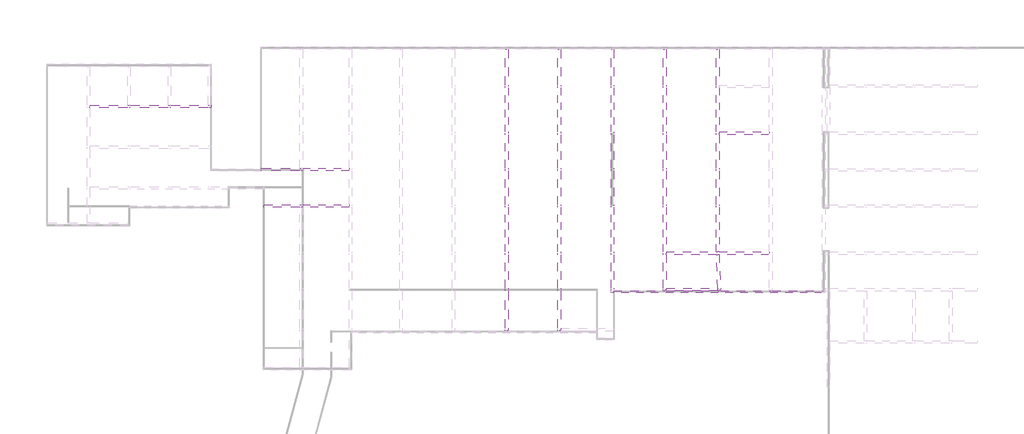
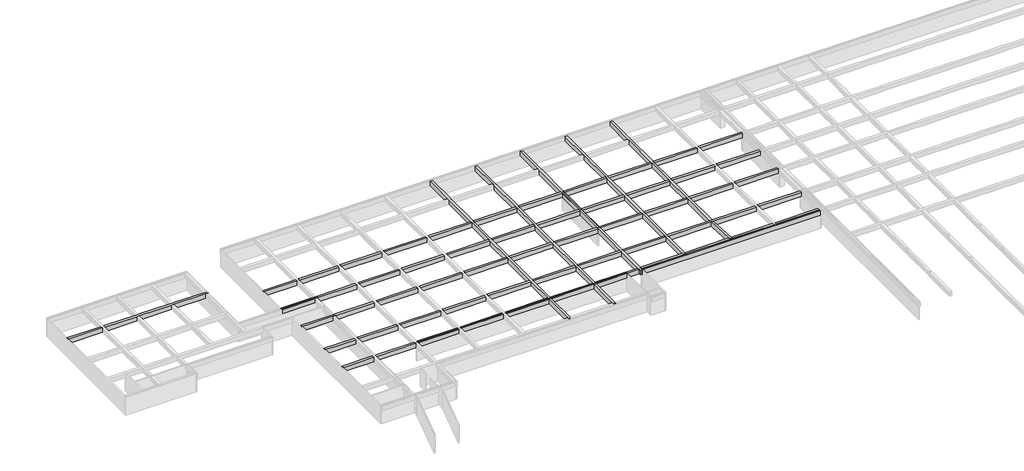
# One storey, part 5 of 14: 13 beams.
"""IFC4 building model written with IfcOpenShell, lengths in millimetres."""

from ifc_helpers import new_model, si_unit, frame, origin, place, context, project, spatial, polyline, outline, extrude, faceted_brep, element, save

model = new_model("IFC4")

# Units and contexts
model_context = context("Model", 3, world=origin())
ifc_project = project(units=[si_unit("LENGTHUNIT", "METRE", prefix="MILLI")], contexts=[model_context])

# Site, building, storey
site = spatial("IfcSite", under=ifc_project)
building = spatial("IfcBuilding", under=site)
storey = spatial("IfcBuildingStorey", under=building, Name="户型图", Elevation=0.0)

# Beams
placement = place(None, origin())
element("IfcBeam", 1, ObjectType="混凝土 - 矩形梁 : KL_beam", at=placement, inside=storey, context=model_context, shape_type="Brep", body=[
    faceted_brep([(-77750.8485237, -125836.5894684, 3300.0), (-77750.8485237, -126236.5894684, 3300.0), (-77750.8485237, -126236.5894684, 2500.0), (-77750.8485237, -125836.5894684, 2500.0), (-77800.8485237, -125836.5894684, 3300.0), (-78200.8485237, -125836.5894684, 3300.0), (-83675.8485237, -125836.5894684, 3300.0), (-84075.8485237, -125836.5894684, 3300.0), (-89675.8485237, -125836.5894684, 3300.0), (-90075.8485237, -125836.5894684, 3300.0), (-95664.0025134, -125836.5894684, 3300.0), (-95664.0025134, -126236.5894684, 3300.0), (-90075.8485237, -126236.5894684, 3300.0), (-89675.8485237, -126236.5894684, 3300.0), (-84075.8485237, -126236.5894684, 3300.0), (-83675.8485237, -126236.5894684, 3300.0), (-78200.8485237, -126236.5894684, 3300.0), (-77800.8485237, -126236.5894684, 3300.0), (-95664.0025134, -126236.5894684, 2500.0), (-90075.8485237, -126236.5894684, 2500.0), (-89675.8485237, -126236.5894684, 2500.0), (-84075.8485237, -126236.5894684, 2500.0), (-83675.8485237, -126236.5894684, 2500.0), (-78200.8485237, -126236.5894684, 2500.0), (-77800.8485237, -126236.5894684, 2500.0), (-95664.0025134, -125836.5894684, 2500.0), (-90075.8485237, -125836.5894684, 2500.0), (-89675.8485237, -125836.5894684, 2500.0), (-84075.8485237, -125836.5894684, 2500.0), (-83675.8485237, -125836.5894684, 2500.0), (-78200.8485237, -125836.5894684, 2500.0), (-77800.8485237, -125836.5894684, 2500.0)], [[[0, 1, 2, 3]], [[1, 0, 4, 5, 6, 7, 8, 9, 10, 11, 12, 13, 14, 15, 16, 17]], [[2, 1, 17, 16, 15, 14, 13, 12, 11, 18, 19, 20, 21, 22, 23, 24]], [[3, 2, 24, 23, 22, 21, 20, 19, 18, 25, 26, 27, 28, 29, 30, 31]], [[0, 3, 31, 30, 29, 28, 27, 26, 25, 10, 9, 8, 7, 6, 5, 4]], [[11, 10, 25, 18]]]),
    faceted_brep([(-102000.8485237, -125836.5894684, 3300.0), (-102000.8485237, -125836.5894684, 2500.0), (-102000.8485237, -126236.5894684, 2500.0), (-102000.8485237, -126236.5894684, 3300.0), (-96064.0025134, -125836.5894684, 3300.0), (-96064.0025134, -126236.5894684, 3300.0), (-96064.0025134, -126236.5894684, 2500.0), (-96064.0025134, -125836.5894684, 2500.0)], [[[0, 1, 2, 3]], [[4, 5, 6, 7]], [[0, 3, 5, 4]], [[3, 2, 6, 5]], [[2, 1, 7, 6]], [[1, 0, 4, 7]]]),
])
element("IfcBeam", 2, ObjectType="混凝土 - 矩形梁 : KL_beam", at=placement, inside=storey, context=model_context, shape_type="Brep", body=[
    faceted_brep([(-34272.7050956, -159158.4277999, 3300.0), (-33872.7050956, -159158.4277999, 3300.0), (-33872.7050956, -158807.3751505, 3300.0), (-33872.7050956, -153248.950757, 3300.0), (-33872.7050956, -152848.950757, 3300.0), (-33872.7050956, -147899.284307, 3300.0), (-33872.7050956, -147499.284307, 3300.0), (-33872.7050956, -140920.0179086, 3300.0), (-33872.7050956, -140520.0179086, 3300.0), (-33872.7050956, -135526.4975491, 3300.0), (-33872.7050956, -135126.4975491, 3300.0), (-33872.7050956, -130180.0179086, 3300.0), (-33872.7050956, -129780.0179086, 3300.0), (-33872.7050956, -123258.950757, 3300.0), (-33872.7050956, -122858.950757, 3300.0), (-33872.7050956, -117558.950757, 3300.0), (-34272.7050956, -117558.950757, 3300.0), (-34272.7050956, -122858.950757, 3300.0), (-34272.7050956, -123258.950757, 3300.0), (-34272.7050956, -129780.0179086, 3300.0), (-34272.7050956, -130180.0179086, 3300.0), (-34272.7050956, -135126.4975491, 3300.0), (-34272.7050956, -135526.4975491, 3300.0), (-34272.7050956, -140520.0179086, 3300.0), (-34272.7050956, -140920.0179086, 3300.0), (-34272.7050956, -147499.284307, 3300.0), (-34272.7050956, -147899.284307, 3300.0), (-34272.7050956, -152848.950757, 3300.0), (-34272.7050956, -153248.950757, 3300.0), (-34272.7050956, -158807.3751505, 3300.0), (-34272.7050956, -159158.4277999, 2500.0), (-34272.7050956, -117558.950757, 2500.0), (-34272.7050956, -122858.950757, 2500.0), (-34272.7050956, -123258.950757, 2500.0), (-34272.7050956, -129780.0179086, 2500.0), (-34272.7050956, -130180.0179086, 2500.0), (-34272.7050956, -135126.4975491, 2500.0), (-34272.7050956, -135526.4975491, 2500.0), (-34272.7050956, -140520.0179086, 2500.0), (-34272.7050956, -140920.0179086, 2500.0), (-34272.7050956, -147499.284307, 2500.0), (-34272.7050956, -147899.284307, 2500.0), (-34272.7050956, -152848.950757, 2500.0), (-34272.7050956, -153248.950757, 2500.0), (-34272.7050956, -158807.3751505, 2500.0), (-33872.7050956, -159158.4277999, 2500.0), (-33872.7050956, -117558.950757, 2500.0), (-33872.7050956, -122858.950757, 2500.0), (-33872.7050956, -123258.950757, 2500.0), (-33872.7050956, -129780.0179086, 2500.0), (-33872.7050956, -130180.0179086, 2500.0), (-33872.7050956, -135126.4975491, 2500.0), (-33872.7050956, -135526.4975491, 2500.0), (-33872.7050956, -140520.0179086, 2500.0), (-33872.7050956, -140920.0179086, 2500.0), (-33872.7050956, -147499.284307, 2500.0), (-33872.7050956, -147899.284307, 2500.0), (-33872.7050956, -152848.950757, 2500.0), (-33872.7050956, -153248.950757, 2500.0), (-33872.7050956, -158807.3751505, 2500.0)], [[[0, 1, 2, 3, 4, 5, 6, 7, 8, 9, 10, 11, 12, 13, 14, 15, 16, 17, 18, 19, 20, 21, 22, 23, 24, 25, 26, 27, 28, 29]], [[30, 0, 29, 28, 27, 26, 25, 24, 23, 22, 21, 20, 19, 18, 17, 16, 31, 32, 33, 34, 35, 36, 37, 38, 39, 40, 41, 42, 43, 44]], [[45, 30, 44, 43, 42, 41, 40, 39, 38, 37, 36, 35, 34, 33, 32, 31, 46, 47, 48, 49, 50, 51, 52, 53, 54, 55, 56, 57, 58, 59]], [[1, 45, 59, 58, 57, 56, 55, 54, 53, 52, 51, 50, 49, 48, 47, 46, 15, 14, 13, 12, 11, 10, 9, 8, 7, 6, 5, 4, 3, 2]], [[1, 0, 30, 45]], [[16, 15, 46, 31]]]),
])
element("IfcBeam", 3, ObjectType="混凝土 - 矩形梁 : KL_beam", at=placement, inside=storey, context=model_context, shape_type="Brep", body=[
    faceted_brep([(-26492.7050956, -159158.4277999, 3300.0), (-26092.7050956, -159158.4277999, 3300.0), (-26092.7050956, -158807.3751505, 3300.0), (-26092.7050956, -153248.950757, 3300.0), (-26092.7050956, -152848.950757, 3300.0), (-26092.7050956, -147899.284307, 3300.0), (-26092.7050956, -147499.284307, 3300.0), (-26092.7050956, -140920.0179086, 3300.0), (-26092.7050956, -140520.0179086, 3300.0), (-26092.7050956, -135526.4975491, 3300.0), (-26092.7050956, -135126.4975491, 3300.0), (-26092.7050956, -130180.0179086, 3300.0), (-26092.7050956, -129780.0179086, 3300.0), (-26092.7050956, -123258.950757, 3300.0), (-26092.7050956, -122858.950757, 3300.0), (-26092.7050956, -117558.950757, 3300.0), (-26492.7050956, -117558.950757, 3300.0), (-26492.7050956, -122858.950757, 3300.0), (-26492.7050956, -123258.950757, 3300.0), (-26492.7050956, -129780.0179086, 3300.0), (-26492.7050956, -130180.0179086, 3300.0), (-26492.7050956, -135126.4975491, 3300.0), (-26492.7050956, -135526.4975491, 3300.0), (-26492.7050956, -140520.0179086, 3300.0), (-26492.7050956, -140920.0179086, 3300.0), (-26492.7050956, -147499.284307, 3300.0), (-26492.7050956, -147899.284307, 3300.0), (-26492.7050956, -152848.950757, 3300.0), (-26492.7050956, -153248.950757, 3300.0), (-26492.7050956, -158807.3751505, 3300.0), (-26092.7050956, -159158.4277999, 2500.0), (-26092.7050956, -158807.3751505, 2500.0), (-26092.7050956, -153248.950757, 2500.0), (-26092.7050956, -152848.950757, 2500.0), (-26092.7050956, -147899.284307, 2500.0), (-26092.7050956, -147499.284307, 2500.0), (-26092.7050956, -140920.0179086, 2500.0), (-26092.7050956, -140520.0179086, 2500.0), (-26092.7050956, -135526.4975491, 2500.0), (-26092.7050956, -135126.4975491, 2500.0), (-26092.7050956, -130180.0179086, 2500.0), (-26092.7050956, -129780.0179086, 2500.0), (-26092.7050956, -123258.950757, 2500.0), (-26092.7050956, -122858.950757, 2500.0), (-26092.7050956, -117558.950757, 2500.0), (-26492.7050956, -159158.4277999, 2500.0), (-26492.7050956, -158807.3751505, 2500.0), (-26492.7050956, -153248.950757, 2500.0), (-26492.7050956, -152848.950757, 2500.0), (-26492.7050956, -147899.284307, 2500.0), (-26492.7050956, -147499.284307, 2500.0), (-26492.7050956, -140920.0179086, 2500.0), (-26492.7050956, -140520.0179086, 2500.0), (-26492.7050956, -135526.4975491, 2500.0), (-26492.7050956, -135126.4975491, 2500.0), (-26492.7050956, -130180.0179086, 2500.0), (-26492.7050956, -129780.0179086, 2500.0), (-26492.7050956, -123258.950757, 2500.0), (-26492.7050956, -122858.950757, 2500.0), (-26492.7050956, -117558.950757, 2500.0)], [[[0, 1, 2, 3, 4, 5, 6, 7, 8, 9, 10, 11, 12, 13, 14, 15, 16, 17, 18, 19, 20, 21, 22, 23, 24, 25, 26, 27, 28, 29]], [[1, 30, 31, 32, 33, 34, 35, 36, 37, 38, 39, 40, 41, 42, 43, 44, 15, 14, 13, 12, 11, 10, 9, 8, 7, 6, 5, 4, 3, 2]], [[30, 45, 46, 47, 48, 49, 50, 51, 52, 53, 54, 55, 56, 57, 58, 59, 44, 43, 42, 41, 40, 39, 38, 37, 36, 35, 34, 33, 32, 31]], [[45, 0, 29, 28, 27, 26, 25, 24, 23, 22, 21, 20, 19, 18, 17, 16, 59, 58, 57, 56, 55, 54, 53, 52, 51, 50, 49, 48, 47, 46]], [[1, 0, 45, 30]], [[16, 15, 44, 59]]]),
])
element("IfcBeam", 4, ObjectType="混凝土 - 矩形梁 : KL_beam", at=placement, inside=storey, context=model_context, shape_type="Brep", body=[
    faceted_brep([(-18655.2993912, -153567.1629538, 3300.0), (-18255.2993912, -153567.1629538, 3300.0), (-18255.2993912, -153248.950757, 3300.0), (-18255.2993912, -152848.950757, 3300.0), (-18255.2993912, -147899.284307, 3300.0), (-18255.2993912, -147499.284307, 3300.0), (-18255.2993912, -140920.0179086, 3300.0), (-18255.2993912, -140520.0179086, 3300.0), (-18255.2993912, -135526.4975491, 3300.0), (-18255.2993912, -135126.4975491, 3300.0), (-18255.2993912, -130180.0179086, 3300.0), (-18255.2993912, -129780.0179086, 3300.0), (-18255.2993912, -123258.950757, 3300.0), (-18255.2993912, -122858.950757, 3300.0), (-18255.2993912, -117558.950757, 3300.0), (-18655.2993912, -117558.950757, 3300.0), (-18655.2993912, -122858.950757, 3300.0), (-18655.2993912, -123258.950757, 3300.0), (-18655.2993912, -129780.0179086, 3300.0), (-18655.2993912, -130180.0179086, 3300.0), (-18655.2993912, -135126.4975491, 3300.0), (-18655.2993912, -135526.4975491, 3300.0), (-18655.2993912, -140520.0179086, 3300.0), (-18655.2993912, -140920.0179086, 3300.0), (-18655.2993912, -147499.284307, 3300.0), (-18655.2993912, -147899.284307, 3300.0), (-18655.2993912, -152848.950757, 3300.0), (-18655.2993912, -153248.950757, 3300.0), (-18655.2993912, -153567.1629538, 2500.0), (-18655.2993912, -117558.950757, 2500.0), (-18655.2993912, -122858.950757, 2500.0), (-18655.2993912, -123258.950757, 2500.0), (-18655.2993912, -129780.0179086, 2500.0), (-18655.2993912, -130180.0179086, 2500.0), (-18655.2993912, -135126.4975491, 2500.0), (-18655.2993912, -135526.4975491, 2500.0), (-18655.2993912, -140520.0179086, 2500.0), (-18655.2993912, -140920.0179086, 2500.0), (-18655.2993912, -147499.284307, 2500.0), (-18655.2993912, -147899.284307, 2500.0), (-18655.2993912, -152848.950757, 2500.0), (-18655.2993912, -153248.950757, 2500.0), (-18255.2993912, -153567.1629538, 2500.0), (-18255.2993912, -117558.950757, 2500.0), (-18255.2993912, -122858.950757, 2500.0), (-18255.2993912, -123258.950757, 2500.0), (-18255.2993912, -129780.0179086, 2500.0), (-18255.2993912, -130180.0179086, 2500.0), (-18255.2993912, -135126.4975491, 2500.0), (-18255.2993912, -135526.4975491, 2500.0), (-18255.2993912, -140520.0179086, 2500.0), (-18255.2993912, -140920.0179086, 2500.0), (-18255.2993912, -147499.284307, 2500.0), (-18255.2993912, -147899.284307, 2500.0), (-18255.2993912, -152848.950757, 2500.0), (-18255.2993912, -153248.950757, 2500.0)], [[[0, 1, 2, 3, 4, 5, 6, 7, 8, 9, 10, 11, 12, 13, 14, 15, 16, 17, 18, 19, 20, 21, 22, 23, 24, 25, 26, 27]], [[28, 0, 27, 26, 25, 24, 23, 22, 21, 20, 19, 18, 17, 16, 15, 29, 30, 31, 32, 33, 34, 35, 36, 37, 38, 39, 40, 41]], [[42, 28, 41, 40, 39, 38, 37, 36, 35, 34, 33, 32, 31, 30, 29, 43, 44, 45, 46, 47, 48, 49, 50, 51, 52, 53, 54, 55]], [[1, 42, 55, 54, 53, 52, 51, 50, 49, 48, 47, 46, 45, 44, 43, 14, 13, 12, 11, 10, 9, 8, 7, 6, 5, 4, 3, 2]], [[1, 0, 28, 42]], [[15, 14, 43, 29]]]),
])
element("IfcBeam", 5, ObjectType="混凝土 - 矩形梁 : KL_beam", at=placement, inside=storey, context=model_context, shape_type="Brep", body=[
    faceted_brep([(-10914.1452268, -153167.1629538, 3300.0), (-10514.1452268, -153167.1629538, 3300.0), (-10514.1452268, -152848.950757, 3300.0), (-10514.1452268, -147899.284307, 3300.0), (-10514.1452268, -147499.284307, 3300.0), (-10514.1452268, -140920.0179086, 3300.0), (-10514.1452268, -140520.0179086, 3300.0), (-10514.1452268, -135526.4975491, 3300.0), (-10514.1452268, -135126.4975491, 3300.0), (-10514.1452268, -130180.0179086, 3300.0), (-10514.1452268, -129780.0179086, 3300.0), (-10514.1452268, -123258.950757, 3300.0), (-10514.1452268, -122858.950757, 3300.0), (-10514.1452268, -117558.950757, 3300.0), (-10914.1452268, -117558.950757, 3300.0), (-10914.1452268, -122858.950757, 3300.0), (-10914.1452268, -123258.950757, 3300.0), (-10914.1452268, -129780.0179086, 3300.0), (-10914.1452268, -130180.0179086, 3300.0), (-10914.1452268, -135126.4975491, 3300.0), (-10914.1452268, -135526.4975491, 3300.0), (-10914.1452268, -140520.0179086, 3300.0), (-10914.1452268, -140920.0179086, 3300.0), (-10914.1452268, -147499.284307, 3300.0), (-10914.1452268, -147899.284307, 3300.0), (-10914.1452268, -152848.950757, 3300.0), (-10914.1452268, -153167.1629538, 2500.0), (-10914.1452268, -117558.950757, 2500.0), (-10914.1452268, -122858.950757, 2500.0), (-10914.1452268, -123258.950757, 2500.0), (-10914.1452268, -129780.0179086, 2500.0), (-10914.1452268, -130180.0179086, 2500.0), (-10914.1452268, -135126.4975491, 2500.0), (-10914.1452268, -135526.4975491, 2500.0), (-10914.1452268, -140520.0179086, 2500.0), (-10914.1452268, -140920.0179086, 2500.0), (-10914.1452268, -147499.284307, 2500.0), (-10914.1452268, -147899.284307, 2500.0), (-10914.1452268, -152848.950757, 2500.0), (-10514.1452268, -153167.1629538, 2500.0), (-10514.1452268, -117558.950757, 2500.0), (-10514.1452268, -122858.950757, 2500.0), (-10514.1452268, -123258.950757, 2500.0), (-10514.1452268, -129780.0179086, 2500.0), (-10514.1452268, -130180.0179086, 2500.0), (-10514.1452268, -135126.4975491, 2500.0), (-10514.1452268, -135526.4975491, 2500.0), (-10514.1452268, -140520.0179086, 2500.0), (-10514.1452268, -140920.0179086, 2500.0), (-10514.1452268, -147499.284307, 2500.0), (-10514.1452268, -147899.284307, 2500.0), (-10514.1452268, -152848.950757, 2500.0)], [[[0, 1, 2, 3, 4, 5, 6, 7, 8, 9, 10, 11, 12, 13, 14, 15, 16, 17, 18, 19, 20, 21, 22, 23, 24, 25]], [[26, 0, 25, 24, 23, 22, 21, 20, 19, 18, 17, 16, 15, 14, 27, 28, 29, 30, 31, 32, 33, 34, 35, 36, 37, 38]], [[39, 26, 38, 37, 36, 35, 34, 33, 32, 31, 30, 29, 28, 27, 40, 41, 42, 43, 44, 45, 46, 47, 48, 49, 50, 51]], [[1, 39, 51, 50, 49, 48, 47, 46, 45, 44, 43, 42, 41, 40, 13, 12, 11, 10, 9, 8, 7, 6, 5, 4, 3, 2]], [[1, 0, 26, 39]], [[14, 13, 40, 27]]]),
])
element("IfcBeam", 6, ObjectType="混凝土 - 矩形梁 : KL_beam", at=placement, inside=storey, context=model_context, shape_type="Brep", body=[
    faceted_brep([(-2680.6534407, -147899.284307, 3300.0), (-3081.0325897, -147899.284307, 3300.0), (-2865.4722954, -152848.950757, 3300.0), (-2851.6140051, -153167.1629538, 3300.0), (-2451.2348561, -153167.1629538, 3300.0), (-2465.0931464, -152848.950757, 3300.0), (-2680.6534407, -147899.284307, 2500.0), (-2451.2348561, -153167.1629538, 2500.0), (-2465.0931464, -152848.950757, 2500.0), (-3081.0325897, -147899.284307, 2500.0), (-2851.6140051, -153167.1629538, 2500.0), (-2865.4722954, -152848.950757, 2500.0)], [[[0, 1, 2, 3, 4, 5]], [[6, 0, 5, 4, 7, 8]], [[9, 6, 8, 7, 10, 11]], [[1, 9, 11, 10, 3, 2]], [[1, 0, 6, 9]], [[4, 3, 10, 7]]]),
])
element("IfcBeam", 7, ObjectType="混凝土 - 矩形梁 : KL_beam", at=placement, inside=storey, context=model_context, shape_type="Brep", body=[
    faceted_brep([(-2691.5778774, -147499.284307, 3300.0), (-2691.5778774, -147499.284307, 2500.0), (-2691.5778774, -140920.0179086, 2500.0), (-2691.5778774, -140520.0179086, 2500.0), (-2691.5778774, -135526.4975491, 2500.0), (-2691.5778774, -135126.4975491, 2500.0), (-2691.5778774, -130180.0179086, 2500.0), (-2691.5778774, -129780.0179086, 2500.0), (-2691.5778774, -123258.950757, 2500.0), (-2691.5778774, -122858.950757, 2500.0), (-2691.5778774, -117558.950757, 2500.0), (-2691.5778774, -117558.950757, 3300.0), (-2691.5778774, -122858.950757, 3300.0), (-2691.5778774, -123258.950757, 3300.0), (-2691.5778774, -129780.0179086, 3300.0), (-2691.5778774, -130180.0179086, 3300.0), (-2691.5778774, -135126.4975491, 3300.0), (-2691.5778774, -135526.4975491, 3300.0), (-2691.5778774, -140520.0179086, 3300.0), (-2691.5778774, -140920.0179086, 3300.0), (-3091.5778774, -147499.284307, 3300.0), (-3091.5778774, -147499.284307, 2500.0), (-3091.5778774, -117558.950757, 3300.0), (-3091.5778774, -122858.950757, 3300.0), (-3091.5778774, -123258.950757, 3300.0), (-3091.5778774, -129780.0179086, 3300.0), (-3091.5778774, -130180.0179086, 3300.0), (-3091.5778774, -135126.4975491, 3300.0), (-3091.5778774, -135526.4975491, 3300.0), (-3091.5778774, -140520.0179086, 3300.0), (-3091.5778774, -140920.0179086, 3300.0), (-3091.5778774, -140920.0179086, 2500.0), (-3091.5778774, -140520.0179086, 2500.0), (-3091.5778774, -135526.4975491, 2500.0), (-3091.5778774, -135126.4975491, 2500.0), (-3091.5778774, -130180.0179086, 2500.0), (-3091.5778774, -129780.0179086, 2500.0), (-3091.5778774, -123258.950757, 2500.0), (-3091.5778774, -122858.950757, 2500.0), (-3091.5778774, -117558.950757, 2500.0)], [[[0, 1, 2, 3, 4, 5, 6, 7, 8, 9, 10, 11, 12, 13, 14, 15, 16, 17, 18, 19]], [[20, 21, 1, 0]], [[20, 0, 19, 18, 17, 16, 15, 14, 13, 12, 11, 22, 23, 24, 25, 26, 27, 28, 29, 30]], [[1, 21, 31, 32, 33, 34, 35, 36, 37, 38, 39, 10, 9, 8, 7, 6, 5, 4, 3, 2]], [[21, 20, 30, 29, 28, 27, 26, 25, 24, 23, 22, 39, 38, 37, 36, 35, 34, 33, 32, 31]], [[11, 10, 39, 22]]]),
])
element("IfcBeam", 8, ObjectType="混凝土 - 矩形梁 : KL_beam", at=placement, inside=storey, context=model_context, shape_type="SweptSolid", body=[
    extrude(outline(polyline([(-70372.7050956, -130180.0179086), (-70372.7050956, -129780.0179086), (-64612.7050956, -129780.0179086), (-64612.7050956, -130180.0179086), (-70372.7050956, -130180.0179086)])), frame((0.0, 0.0, 2500.0), z_axis=(0.0, 0.0, 1.0), x_axis=(1.0, 0.0, 0.0)), (0.0, 0.0, 1.0), 800.0),
    extrude(outline(polyline([(12577.2949044, -129780.0179086), (12577.2949044, -130180.0179086), (5154.7716095, -130180.0179086), (5154.7716095, -129780.0179086), (12577.2949044, -129780.0179086)])), frame((0.0, 0.0, 2500.0), z_axis=(0.0, 0.0, 1.0), x_axis=(1.0, 0.0, 0.0)), (0.0, 0.0, 1.0), 800.0),
    extrude(outline(polyline([(-64212.7050956, -130180.0179086), (-64212.7050956, -129780.0179086), (-57355.3281677, -129780.0179086), (-57355.3281677, -130180.0179086), (-64212.7050956, -130180.0179086)])), frame((0.0, 0.0, 2500.0), z_axis=(0.0, 0.0, 1.0), x_axis=(1.0, 0.0, 0.0)), (0.0, 0.0, 1.0), 800.0),
    extrude(outline(polyline([(-56955.3281677, -130180.0179086), (-56955.3281677, -129780.0179086), (-49869.9201432, -129780.0179086), (-49869.9201432, -130180.0179086), (-56955.3281677, -130180.0179086)])), frame((0.0, 0.0, 2500.0), z_axis=(0.0, 0.0, 1.0), x_axis=(1.0, 0.0, 0.0)), (0.0, 0.0, 1.0), 800.0),
    extrude(outline(polyline([(-49469.9201432, -130180.0179086), (-49469.9201432, -129780.0179086), (-42115.0194088, -129780.0179086), (-42115.0194088, -130180.0179086), (-49469.9201432, -130180.0179086)])), frame((0.0, 0.0, 2500.0), z_axis=(0.0, 0.0, 1.0), x_axis=(1.0, 0.0, 0.0)), (0.0, 0.0, 1.0), 800.0),
    extrude(outline(polyline([(-41715.0194088, -130180.0179086), (-41715.0194088, -129780.0179086), (-34272.7050956, -129780.0179086), (-34272.7050956, -130180.0179086), (-41715.0194088, -130180.0179086)])), frame((0.0, 0.0, 2500.0), z_axis=(0.0, 0.0, 1.0), x_axis=(1.0, 0.0, 0.0)), (0.0, 0.0, 1.0), 800.0),
    extrude(outline(polyline([(-33872.7050956, -130180.0179086), (-33872.7050956, -129780.0179086), (-26492.7050956, -129780.0179086), (-26492.7050956, -130180.0179086), (-33872.7050956, -130180.0179086)])), frame((0.0, 0.0, 2500.0), z_axis=(0.0, 0.0, 1.0), x_axis=(1.0, 0.0, 0.0)), (0.0, 0.0, 1.0), 800.0),
    extrude(outline(polyline([(-26092.7050956, -130180.0179086), (-26092.7050956, -129780.0179086), (-18655.2993912, -129780.0179086), (-18655.2993912, -130180.0179086), (-26092.7050956, -130180.0179086)])), frame((0.0, 0.0, 2500.0), z_axis=(0.0, 0.0, 1.0), x_axis=(1.0, 0.0, 0.0)), (0.0, 0.0, 1.0), 800.0),
    extrude(outline(polyline([(-18255.2993912, -130180.0179086), (-18255.2993912, -129780.0179086), (-10914.1452268, -129780.0179086), (-10914.1452268, -130180.0179086), (-18255.2993912, -130180.0179086)])), frame((0.0, 0.0, 2500.0), z_axis=(0.0, 0.0, 1.0), x_axis=(1.0, 0.0, 0.0)), (0.0, 0.0, 1.0), 800.0),
    extrude(outline(polyline([(-10514.1452268, -130180.0179086), (-10514.1452268, -129780.0179086), (-3091.5778774, -129780.0179086), (-3091.5778774, -130180.0179086), (-10514.1452268, -130180.0179086)])), frame((0.0, 0.0, 2500.0), z_axis=(0.0, 0.0, 1.0), x_axis=(1.0, 0.0, 0.0)), (0.0, 0.0, 1.0), 800.0),
    extrude(outline(polyline([(-2691.5778774, -130180.0179086), (-2691.5778774, -129780.0179086), (4754.7716095, -129780.0179086), (4754.7716095, -130180.0179086), (-2691.5778774, -130180.0179086)])), frame((0.0, 0.0, 2500.0), z_axis=(0.0, 0.0, 1.0), x_axis=(1.0, 0.0, 0.0)), (0.0, 0.0, 1.0), 800.0),
])
element("IfcBeam", 9, ObjectType="混凝土 - 矩形梁 : KL_beam", at=placement, inside=storey, context=model_context, shape_type="Brep", body=[
    faceted_brep([(-57355.3281677, -135126.4975491, 3300.0), (-64212.7050956, -135126.4975491, 3300.0), (-64612.7050956, -135126.4975491, 3300.0), (-70313.0159659, -135126.4975491, 3300.0), (-70313.0159659, -135208.950757, 3300.0), (-70313.0159659, -135526.4975491, 3300.0), (-64612.7050956, -135526.4975491, 3300.0), (-64212.7050956, -135526.4975491, 3300.0), (-57355.3281677, -135526.4975491, 3300.0), (-70313.0159659, -135526.4975491, 2500.0), (-64612.7050956, -135526.4975491, 2500.0), (-64212.7050956, -135526.4975491, 2500.0), (-57355.3281677, -135526.4975491, 2500.0), (-70313.0159659, -135208.950757, 2500.0), (-70313.0159659, -135126.4975491, 2500.0), (-64612.7050956, -135126.4975491, 2500.0), (-64212.7050956, -135126.4975491, 2500.0), (-57355.3281677, -135126.4975491, 2500.0)], [[[0, 1, 2, 3, 4, 5, 6, 7, 8]], [[8, 7, 6, 5, 9, 10, 11, 12]], [[12, 11, 10, 9, 13, 14, 15, 16, 17]], [[3, 2, 1, 0, 17, 16, 15, 14]], [[0, 8, 12, 17]], [[3, 14, 13, 9, 5, 4]]]),
    faceted_brep([(12577.2949044, -135126.4975491, 3300.0), (12577.2949044, -135526.4975491, 3300.0), (12577.2949044, -135526.4975491, 2500.0), (12577.2949044, -135126.4975491, 2500.0), (5154.7716095, -135526.4975491, 3300.0), (5154.7716095, -135126.4975491, 3300.0), (5154.7716095, -135126.4975491, 2500.0), (5154.7716095, -135526.4975491, 2500.0)], [[[0, 1, 2, 3]], [[4, 5, 6, 7]], [[1, 0, 5, 4]], [[2, 1, 4, 7]], [[3, 2, 7, 6]], [[0, 3, 6, 5]]]),
    faceted_brep([(-56955.3281677, -135526.4975491, 3300.0), (-56955.3281677, -135126.4975491, 3300.0), (-56955.3281677, -135126.4975491, 2500.0), (-56955.3281677, -135526.4975491, 2500.0), (-49869.9201432, -135126.4975491, 3300.0), (-49869.9201432, -135526.4975491, 3300.0), (-49869.9201432, -135526.4975491, 2500.0), (-49869.9201432, -135126.4975491, 2500.0)], [[[0, 1, 2, 3]], [[4, 5, 6, 7]], [[1, 0, 5, 4]], [[0, 3, 6, 5]], [[3, 2, 7, 6]], [[2, 1, 4, 7]]]),
    faceted_brep([(-42115.0194088, -135126.4975491, 3300.0), (-49469.9201432, -135126.4975491, 3300.0), (-49469.9201432, -135526.4975491, 3300.0), (-42115.0194088, -135526.4975491, 3300.0), (-49469.9201432, -135526.4975491, 2500.0), (-42115.0194088, -135526.4975491, 2500.0), (-49469.9201432, -135126.4975491, 2500.0), (-42115.0194088, -135126.4975491, 2500.0)], [[[0, 1, 2, 3]], [[3, 2, 4, 5]], [[5, 4, 6, 7]], [[1, 0, 7, 6]], [[2, 1, 6, 4]], [[0, 3, 5, 7]]]),
    faceted_brep([(-41715.0194088, -135526.4975491, 3300.0), (-41715.0194088, -135126.4975491, 3300.0), (-41715.0194088, -135126.4975491, 2500.0), (-41715.0194088, -135526.4975491, 2500.0), (-34272.7050956, -135126.4975491, 3300.0), (-34272.7050956, -135526.4975491, 3300.0), (-34272.7050956, -135526.4975491, 2500.0), (-34272.7050956, -135126.4975491, 2500.0)], [[[0, 1, 2, 3]], [[4, 5, 6, 7]], [[4, 1, 0, 5]], [[5, 0, 3, 6]], [[6, 3, 2, 7]], [[1, 4, 7, 2]]]),
    faceted_brep([(-33872.7050956, -135526.4975491, 3300.0), (-33872.7050956, -135126.4975491, 3300.0), (-33872.7050956, -135126.4975491, 2500.0), (-33872.7050956, -135526.4975491, 2500.0), (-26492.7050956, -135126.4975491, 3300.0), (-26492.7050956, -135526.4975491, 3300.0), (-26492.7050956, -135526.4975491, 2500.0), (-26492.7050956, -135126.4975491, 2500.0)], [[[0, 1, 2, 3]], [[4, 5, 6, 7]], [[4, 1, 0, 5]], [[5, 0, 3, 6]], [[6, 3, 2, 7]], [[1, 4, 7, 2]]]),
    faceted_brep([(-26092.7050956, -135526.4975491, 3300.0), (-26092.7050956, -135126.4975491, 3300.0), (-26092.7050956, -135126.4975491, 2500.0), (-26092.7050956, -135526.4975491, 2500.0), (-18655.2993912, -135126.4975491, 3300.0), (-18655.2993912, -135526.4975491, 3300.0), (-18655.2993912, -135526.4975491, 2500.0), (-18655.2993912, -135126.4975491, 2500.0)], [[[0, 1, 2, 3]], [[4, 5, 6, 7]], [[4, 1, 0, 5]], [[5, 0, 3, 6]], [[6, 3, 2, 7]], [[1, 4, 7, 2]]]),
    faceted_brep([(-18255.2993912, -135526.4975491, 3300.0), (-18255.2993912, -135126.4975491, 3300.0), (-18255.2993912, -135126.4975491, 2500.0), (-18255.2993912, -135526.4975491, 2500.0), (-10914.1452268, -135126.4975491, 3300.0), (-10914.1452268, -135526.4975491, 3300.0), (-10914.1452268, -135526.4975491, 2500.0), (-10914.1452268, -135126.4975491, 2500.0)], [[[0, 1, 2, 3]], [[4, 5, 6, 7]], [[4, 1, 0, 5]], [[5, 0, 3, 6]], [[6, 3, 2, 7]], [[1, 4, 7, 2]]]),
    faceted_brep([(-10514.1452268, -135526.4975491, 3300.0), (-10514.1452268, -135126.4975491, 3300.0), (-10514.1452268, -135126.4975491, 2500.0), (-10514.1452268, -135526.4975491, 2500.0), (-3091.5778774, -135126.4975491, 3300.0), (-3091.5778774, -135526.4975491, 3300.0), (-3091.5778774, -135526.4975491, 2500.0), (-3091.5778774, -135126.4975491, 2500.0)], [[[0, 1, 2, 3]], [[4, 5, 6, 7]], [[4, 1, 0, 5]], [[5, 0, 3, 6]], [[6, 3, 2, 7]], [[1, 4, 7, 2]]]),
    faceted_brep([(-2691.5778774, -135526.4975491, 3300.0), (-2691.5778774, -135126.4975491, 3300.0), (-2691.5778774, -135126.4975491, 2500.0), (-2691.5778774, -135526.4975491, 2500.0), (4754.7716095, -135126.4975491, 3300.0), (4754.7716095, -135526.4975491, 3300.0), (4754.7716095, -135526.4975491, 2500.0), (4754.7716095, -135126.4975491, 2500.0)], [[[0, 1, 2, 3]], [[4, 5, 6, 7]], [[1, 0, 5, 4]], [[0, 3, 6, 5]], [[3, 2, 7, 6]], [[2, 1, 4, 7]]]),
])
element("IfcBeam", 10, ObjectType="混凝土 - 矩形梁 : KL_beam", at=placement, inside=storey, context=model_context, shape_type="Brep", body=[
    faceted_brep([(-69972.7050956, -140920.0179086, 3300.0), (-69972.7050956, -140520.0179086, 3300.0), (-69972.7050956, -140520.0179086, 2500.0), (-69972.7050956, -140920.0179086, 2500.0), (-64612.7050956, -140920.0179086, 3300.0), (-64212.7050956, -140920.0179086, 3300.0), (-57355.3281677, -140920.0179086, 3300.0), (-57355.3281677, -140520.0179086, 3300.0), (-64212.7050956, -140520.0179086, 3300.0), (-64612.7050956, -140520.0179086, 3300.0), (-57355.3281677, -140520.0179086, 2500.0), (-64212.7050956, -140520.0179086, 2500.0), (-64612.7050956, -140520.0179086, 2500.0), (-57355.3281677, -140920.0179086, 2500.0), (-64212.7050956, -140920.0179086, 2500.0), (-64612.7050956, -140920.0179086, 2500.0)], [[[0, 1, 2, 3]], [[1, 0, 4, 5, 6, 7, 8, 9]], [[2, 1, 9, 8, 7, 10, 11, 12]], [[3, 2, 12, 11, 10, 13, 14, 15]], [[0, 3, 15, 14, 13, 6, 5, 4]], [[7, 6, 13, 10]]]),
    faceted_brep([(12577.2949044, -140520.0179086, 3300.0), (12577.2949044, -140920.0179086, 3300.0), (12577.2949044, -140920.0179086, 2500.0), (12577.2949044, -140520.0179086, 2500.0), (5154.7716095, -140920.0179086, 3300.0), (5154.7716095, -140520.0179086, 3300.0), (5154.7716095, -140520.0179086, 2500.0), (5154.7716095, -140920.0179086, 2500.0)], [[[0, 1, 2, 3]], [[4, 5, 6, 7]], [[1, 0, 5, 4]], [[0, 3, 6, 5]], [[3, 2, 7, 6]], [[2, 1, 4, 7]]]),
    faceted_brep([(-56955.3281677, -140920.0179086, 3300.0), (-56955.3281677, -140520.0179086, 3300.0), (-56955.3281677, -140520.0179086, 2500.0), (-56955.3281677, -140920.0179086, 2500.0), (-49869.9201432, -140920.0179086, 3300.0), (-49869.9201432, -140520.0179086, 3300.0), (-49869.9201432, -140520.0179086, 2500.0), (-49869.9201432, -140920.0179086, 2500.0)], [[[0, 1, 2, 3]], [[1, 0, 4, 5]], [[2, 1, 5, 6]], [[3, 2, 6, 7]], [[0, 3, 7, 4]], [[5, 4, 7, 6]]]),
    faceted_brep([(-49469.9201432, -140920.0179086, 3300.0), (-49469.9201432, -140520.0179086, 3300.0), (-49469.9201432, -140520.0179086, 2500.0), (-49469.9201432, -140920.0179086, 2500.0), (-42115.0194088, -140920.0179086, 3300.0), (-42115.0194088, -140520.0179086, 3300.0), (-42115.0194088, -140520.0179086, 2500.0), (-42115.0194088, -140920.0179086, 2500.0)], [[[0, 1, 2, 3]], [[1, 0, 4, 5]], [[2, 1, 5, 6]], [[3, 2, 6, 7]], [[0, 3, 7, 4]], [[5, 4, 7, 6]]]),
    faceted_brep([(-41715.0194088, -140920.0179086, 3300.0), (-41715.0194088, -140520.0179086, 3300.0), (-41715.0194088, -140520.0179086, 2500.0), (-41715.0194088, -140920.0179086, 2500.0), (-34272.7050956, -140920.0179086, 3300.0), (-34272.7050956, -140520.0179086, 3300.0), (-34272.7050956, -140520.0179086, 2500.0), (-34272.7050956, -140920.0179086, 2500.0)], [[[0, 1, 2, 3]], [[1, 0, 4, 5]], [[2, 1, 5, 6]], [[3, 2, 6, 7]], [[0, 3, 7, 4]], [[5, 4, 7, 6]]]),
    faceted_brep([(-33872.7050956, -140920.0179086, 3300.0), (-33872.7050956, -140520.0179086, 3300.0), (-33872.7050956, -140520.0179086, 2500.0), (-33872.7050956, -140920.0179086, 2500.0), (-26492.7050956, -140920.0179086, 3300.0), (-26492.7050956, -140520.0179086, 3300.0), (-26492.7050956, -140520.0179086, 2500.0), (-26492.7050956, -140920.0179086, 2500.0)], [[[0, 1, 2, 3]], [[1, 0, 4, 5]], [[2, 1, 5, 6]], [[3, 2, 6, 7]], [[0, 3, 7, 4]], [[5, 4, 7, 6]]]),
    faceted_brep([(-26092.7050956, -140920.0179086, 3300.0), (-26092.7050956, -140520.0179086, 3300.0), (-26092.7050956, -140520.0179086, 2500.0), (-26092.7050956, -140920.0179086, 2500.0), (-18655.2993912, -140920.0179086, 3300.0), (-18655.2993912, -140520.0179086, 3300.0), (-18655.2993912, -140520.0179086, 2500.0), (-18655.2993912, -140920.0179086, 2500.0)], [[[0, 1, 2, 3]], [[1, 0, 4, 5]], [[2, 1, 5, 6]], [[3, 2, 6, 7]], [[0, 3, 7, 4]], [[5, 4, 7, 6]]]),
    faceted_brep([(-18255.2993912, -140920.0179086, 3300.0), (-18255.2993912, -140520.0179086, 3300.0), (-18255.2993912, -140520.0179086, 2500.0), (-18255.2993912, -140920.0179086, 2500.0), (-10914.1452268, -140920.0179086, 3300.0), (-10914.1452268, -140520.0179086, 3300.0), (-10914.1452268, -140520.0179086, 2500.0), (-10914.1452268, -140920.0179086, 2500.0)], [[[0, 1, 2, 3]], [[1, 0, 4, 5]], [[2, 1, 5, 6]], [[3, 2, 6, 7]], [[0, 3, 7, 4]], [[5, 4, 7, 6]]]),
    faceted_brep([(-10514.1452268, -140920.0179086, 3300.0), (-10514.1452268, -140520.0179086, 3300.0), (-10514.1452268, -140520.0179086, 2500.0), (-10514.1452268, -140920.0179086, 2500.0), (-3091.5778774, -140920.0179086, 3300.0), (-3091.5778774, -140520.0179086, 3300.0), (-3091.5778774, -140520.0179086, 2500.0), (-3091.5778774, -140920.0179086, 2500.0)], [[[0, 1, 2, 3]], [[1, 0, 4, 5]], [[2, 1, 5, 6]], [[3, 2, 6, 7]], [[0, 3, 7, 4]], [[5, 4, 7, 6]]]),
    faceted_brep([(-2691.5778774, -140920.0179086, 3300.0), (-2691.5778774, -140520.0179086, 3300.0), (-2691.5778774, -140520.0179086, 2500.0), (-2691.5778774, -140920.0179086, 2500.0), (4754.7716095, -140920.0179086, 3300.0), (4754.7716095, -140520.0179086, 3300.0), (4754.7716095, -140520.0179086, 2500.0), (4754.7716095, -140920.0179086, 2500.0)], [[[0, 1, 2, 3]], [[1, 0, 4, 5]], [[2, 1, 5, 6]], [[3, 2, 6, 7]], [[0, 3, 7, 4]], [[5, 4, 7, 6]]]),
])
element("IfcBeam", 11, ObjectType="混凝土 - 矩形梁 : KL_beam", at=placement, inside=storey, context=model_context, shape_type="Brep", body=[
    faceted_brep([(-69972.7050956, -147499.284307, 3300.0), (-69972.7050956, -147499.284307, 2500.0), (-69972.7050956, -147899.284307, 2500.0), (-69972.7050956, -147899.284307, 3300.0), (-64612.7050956, -147499.284307, 3300.0), (-64612.7050956, -147899.284307, 3300.0), (-64612.7050956, -147899.284307, 2500.0), (-64612.7050956, -147499.284307, 2500.0)], [[[0, 1, 2, 3]], [[4, 5, 6, 7]], [[0, 3, 5, 4]], [[3, 2, 6, 5]], [[2, 1, 7, 6]], [[1, 0, 4, 7]]]),
    faceted_brep([(-56955.3281677, -147499.284307, 3300.0), (-56955.3281677, -147899.284307, 3300.0), (-49869.9201432, -147899.284307, 3300.0), (-49869.9201432, -147499.284307, 3300.0), (-56955.3281677, -147899.284307, 2500.0), (-49869.9201432, -147899.284307, 2500.0), (-56955.3281677, -147499.284307, 2500.0), (-49869.9201432, -147499.284307, 2500.0)], [[[0, 1, 2, 3]], [[1, 4, 5, 2]], [[4, 6, 7, 5]], [[6, 0, 3, 7]], [[1, 0, 6, 4]], [[3, 2, 5, 7]]]),
    faceted_brep([(12577.2949044, -147499.284307, 3300.0), (12577.2949044, -147899.284307, 3300.0), (12577.2949044, -147899.284307, 2500.0), (12577.2949044, -147499.284307, 2500.0), (5154.7716095, -147899.284307, 3300.0), (5154.7716095, -147499.284307, 3300.0), (5154.7716095, -147499.284307, 2500.0), (5154.7716095, -147899.284307, 2500.0)], [[[0, 1, 2, 3]], [[4, 5, 6, 7]], [[1, 0, 5, 4]], [[2, 1, 4, 7]], [[3, 2, 7, 6]], [[0, 3, 6, 5]]]),
    faceted_brep([(-57355.3281677, -147499.284307, 3300.0), (-57355.3281677, -147899.284307, 3300.0), (-57355.3281677, -147899.284307, 2500.0), (-57355.3281677, -147499.284307, 2500.0), (-64212.7050956, -147499.284307, 3300.0), (-64212.7050956, -147899.284307, 3300.0), (-64212.7050956, -147899.284307, 2500.0), (-64212.7050956, -147499.284307, 2500.0)], [[[0, 1, 2, 3]], [[1, 0, 4, 5]], [[2, 1, 5, 6]], [[3, 2, 6, 7]], [[0, 3, 7, 4]], [[5, 4, 7, 6]]]),
    faceted_brep([(-49469.9201432, -147899.284307, 3300.0), (-49469.9201432, -147499.284307, 3300.0), (-49469.9201432, -147499.284307, 2500.0), (-49469.9201432, -147899.284307, 2500.0), (-42115.0194088, -147499.284307, 3300.0), (-42115.0194088, -147899.284307, 3300.0), (-42115.0194088, -147899.284307, 2500.0), (-42115.0194088, -147499.284307, 2500.0)], [[[0, 1, 2, 3]], [[4, 5, 6, 7]], [[1, 0, 5, 4]], [[0, 3, 6, 5]], [[3, 2, 7, 6]], [[2, 1, 4, 7]]]),
    faceted_brep([(-41715.0194088, -147499.284307, 3300.0), (-41715.0194088, -147899.284307, 3300.0), (-34272.7050956, -147899.284307, 3300.0), (-34272.7050956, -147499.284307, 3300.0), (-41715.0194088, -147899.284307, 2500.0), (-34272.7050956, -147899.284307, 2500.0), (-41715.0194088, -147499.284307, 2500.0), (-34272.7050956, -147499.284307, 2500.0)], [[[0, 1, 2, 3]], [[1, 4, 5, 2]], [[4, 6, 7, 5]], [[6, 0, 3, 7]], [[1, 0, 6, 4]], [[3, 2, 5, 7]]]),
    faceted_brep([(-33872.7050956, -147899.284307, 3300.0), (-33872.7050956, -147499.284307, 3300.0), (-33872.7050956, -147499.284307, 2500.0), (-33872.7050956, -147899.284307, 2500.0), (-26492.7050956, -147499.284307, 3300.0), (-26492.7050956, -147899.284307, 3300.0), (-26492.7050956, -147899.284307, 2500.0), (-26492.7050956, -147499.284307, 2500.0)], [[[0, 1, 2, 3]], [[4, 5, 6, 7]], [[1, 0, 5, 4]], [[0, 3, 6, 5]], [[3, 2, 7, 6]], [[2, 1, 4, 7]]]),
    faceted_brep([(-26092.7050956, -147499.284307, 3300.0), (-26092.7050956, -147899.284307, 3300.0), (-18655.2993912, -147899.284307, 3300.0), (-18655.2993912, -147499.284307, 3300.0), (-26092.7050956, -147899.284307, 2500.0), (-18655.2993912, -147899.284307, 2500.0), (-26092.7050956, -147499.284307, 2500.0), (-18655.2993912, -147499.284307, 2500.0)], [[[0, 1, 2, 3]], [[1, 4, 5, 2]], [[4, 6, 7, 5]], [[6, 0, 3, 7]], [[1, 0, 6, 4]], [[3, 2, 5, 7]]]),
    faceted_brep([(-18255.2993912, -147899.284307, 3300.0), (-18255.2993912, -147499.284307, 3300.0), (-18255.2993912, -147499.284307, 2500.0), (-18255.2993912, -147899.284307, 2500.0), (-10914.1452268, -147499.284307, 3300.0), (-10914.1452268, -147899.284307, 3300.0), (-10914.1452268, -147899.284307, 2500.0), (-10914.1452268, -147499.284307, 2500.0)], [[[0, 1, 2, 3]], [[4, 5, 6, 7]], [[1, 0, 5, 4]], [[0, 3, 6, 5]], [[3, 2, 7, 6]], [[2, 1, 4, 7]]]),
    faceted_brep([(-10514.1452268, -147499.284307, 3300.0), (-10514.1452268, -147899.284307, 3300.0), (-3081.0325897, -147899.284307, 3300.0), (-2680.6534407, -147899.284307, 3300.0), (4754.7716095, -147899.284307, 3300.0), (4754.7716095, -147499.284307, 3300.0), (-2691.5778774, -147499.284307, 3300.0), (-3091.5778774, -147499.284307, 3300.0), (-10514.1452268, -147899.284307, 2500.0), (-3081.0325897, -147899.284307, 2500.0), (-2680.6534407, -147899.284307, 2500.0), (4754.7716095, -147899.284307, 2500.0), (-10514.1452268, -147499.284307, 2500.0), (-3091.5778774, -147499.284307, 2500.0), (-2691.5778774, -147499.284307, 2500.0), (4754.7716095, -147499.284307, 2500.0)], [[[0, 1, 2, 3, 4, 5, 6, 7]], [[1, 8, 9, 10, 11, 4, 3, 2]], [[8, 12, 13, 14, 15, 11, 10, 9]], [[12, 0, 7, 6, 5, 15, 14, 13]], [[1, 0, 12, 8]], [[5, 4, 11, 15]]]),
])
element("IfcBeam", 12, ObjectType="混凝土 - 矩形梁 : KL_beam", at=placement, inside=storey, context=model_context, shape_type="Brep", body=[
    faceted_brep([(-69972.7050956, -152848.950757, 3300.0), (-69972.7050956, -152848.950757, 2500.0), (-69972.7050956, -153248.950757, 2500.0), (-69972.7050956, -153248.950757, 3300.0), (-64612.7050956, -152848.950757, 3300.0), (-64612.7050956, -153248.950757, 3300.0), (-64612.7050956, -153248.950757, 2500.0), (-64612.7050956, -152848.950757, 2500.0)], [[[0, 1, 2, 3]], [[4, 5, 6, 7]], [[0, 3, 5, 4]], [[3, 2, 6, 5]], [[2, 1, 7, 6]], [[1, 0, 4, 7]]]),
    faceted_brep([(-56955.3281677, -152848.950757, 3300.0), (-56955.3281677, -153248.950757, 3300.0), (-49869.9201432, -153248.950757, 3300.0), (-49869.9201432, -152848.950757, 3300.0), (-56955.3281677, -153248.950757, 2500.0), (-49869.9201432, -153248.950757, 2500.0), (-56955.3281677, -152848.950757, 2500.0), (-49869.9201432, -152848.950757, 2500.0)], [[[0, 1, 2, 3]], [[1, 4, 5, 2]], [[4, 6, 7, 5]], [[6, 0, 3, 7]], [[1, 0, 6, 4]], [[3, 2, 5, 7]]]),
    faceted_brep([(12577.2949044, -152848.950757, 3300.0), (12577.2949044, -153248.950757, 3300.0), (12577.2949044, -153248.950757, 2500.0), (12577.2949044, -152848.950757, 2500.0), (5154.7716095, -152848.950757, 3300.0), (5154.7716095, -153167.1629538, 3300.0), (5154.7716095, -153248.950757, 3300.0), (5154.7716095, -153248.950757, 2500.0), (5154.7716095, -153167.1629538, 2500.0), (5154.7716095, -152848.950757, 2500.0)], [[[0, 1, 2, 3]], [[1, 0, 4, 5, 6]], [[2, 1, 6, 7]], [[3, 2, 7, 8, 9]], [[0, 3, 9, 4]], [[6, 5, 4, 9, 8, 7]]]),
    faceted_brep([(-57355.3281677, -152848.950757, 3300.0), (-57355.3281677, -153248.950757, 3300.0), (-57355.3281677, -153248.950757, 2500.0), (-57355.3281677, -152848.950757, 2500.0), (-64212.7050956, -152848.950757, 3300.0), (-64212.7050956, -153248.950757, 3300.0), (-64212.7050956, -153248.950757, 2500.0), (-64212.7050956, -152848.950757, 2500.0)], [[[0, 1, 2, 3]], [[1, 0, 4, 5]], [[2, 1, 5, 6]], [[3, 2, 6, 7]], [[0, 3, 7, 4]], [[5, 4, 7, 6]]]),
    faceted_brep([(-49469.9201432, -153248.950757, 3300.0), (-49469.9201432, -152848.950757, 3300.0), (-49469.9201432, -152848.950757, 2500.0), (-49469.9201432, -153248.950757, 2500.0), (-42115.0194088, -152848.950757, 3300.0), (-42115.0194088, -153248.950757, 3300.0), (-42115.0194088, -153248.950757, 2500.0), (-42115.0194088, -152848.950757, 2500.0)], [[[0, 1, 2, 3]], [[4, 5, 6, 7]], [[1, 0, 5, 4]], [[0, 3, 6, 5]], [[3, 2, 7, 6]], [[2, 1, 4, 7]]]),
    faceted_brep([(-41715.0194088, -152848.950757, 3300.0), (-41715.0194088, -153248.950757, 3300.0), (-34272.7050956, -153248.950757, 3300.0), (-34272.7050956, -152848.950757, 3300.0), (-41715.0194088, -153248.950757, 2500.0), (-34272.7050956, -153248.950757, 2500.0), (-41715.0194088, -152848.950757, 2500.0), (-34272.7050956, -152848.950757, 2500.0)], [[[0, 1, 2, 3]], [[1, 4, 5, 2]], [[4, 6, 7, 5]], [[6, 0, 3, 7]], [[1, 0, 6, 4]], [[3, 2, 5, 7]]]),
    faceted_brep([(-33872.7050956, -153248.950757, 3300.0), (-33872.7050956, -152848.950757, 3300.0), (-33872.7050956, -152848.950757, 2500.0), (-33872.7050956, -153248.950757, 2500.0), (-26492.7050956, -152848.950757, 3300.0), (-26492.7050956, -153248.950757, 3300.0), (-26492.7050956, -153248.950757, 2500.0), (-26492.7050956, -152848.950757, 2500.0)], [[[0, 1, 2, 3]], [[4, 5, 6, 7]], [[1, 0, 5, 4]], [[0, 3, 6, 5]], [[3, 2, 7, 6]], [[2, 1, 4, 7]]]),
    faceted_brep([(-26092.7050956, -152848.950757, 3300.0), (-26092.7050956, -153248.950757, 3300.0), (-18655.2993912, -153248.950757, 3300.0), (-18655.2993912, -152848.950757, 3300.0), (-26092.7050956, -153248.950757, 2500.0), (-18655.2993912, -153248.950757, 2500.0), (-26092.7050956, -152848.950757, 2500.0), (-18655.2993912, -152848.950757, 2500.0)], [[[0, 1, 2, 3]], [[1, 4, 5, 2]], [[4, 6, 7, 5]], [[6, 0, 3, 7]], [[1, 0, 6, 4]], [[3, 2, 5, 7]]]),
    faceted_brep([(-18255.2993912, -153248.950757, 3300.0), (-18255.2993912, -152848.950757, 3300.0), (-18255.2993912, -152848.950757, 2500.0), (-18255.2993912, -153248.950757, 2500.0), (-10914.1452268, -152848.950757, 3300.0), (-10914.1452268, -153167.1629538, 3300.0), (-10914.1452268, -153248.950757, 3300.0), (-10914.1452268, -153248.950757, 2500.0), (-10914.1452268, -153167.1629538, 2500.0), (-10914.1452268, -152848.950757, 2500.0)], [[[0, 1, 2, 3]], [[4, 5, 6, 7, 8, 9]], [[1, 0, 6, 5, 4]], [[0, 3, 7, 6]], [[3, 2, 9, 8, 7]], [[2, 1, 4, 9]]]),
    faceted_brep([(-10514.1452268, -152848.950757, 3300.0), (-10514.1452268, -153167.1629538, 3300.0), (-10514.1452268, -153248.950757, 3300.0), (-2848.0521079, -153248.950757, 3300.0), (-2851.6140051, -153167.1629538, 3300.0), (-2865.4722954, -152848.950757, 3300.0), (-10514.1452268, -153248.950757, 2500.0), (-2848.0521079, -153248.950757, 2500.0), (-10514.1452268, -153167.1629538, 2500.0), (-10514.1452268, -152848.950757, 2500.0), (-2865.4722954, -152848.950757, 2500.0), (-2851.6140051, -153167.1629538, 2500.0)], [[[0, 1, 2, 3, 4, 5]], [[2, 6, 7, 3]], [[6, 8, 9, 10, 11, 7]], [[9, 0, 5, 10]], [[2, 1, 0, 9, 8, 6]], [[5, 4, 3, 7, 11, 10]]]),
    faceted_brep([(-2447.6729589, -153248.950757, 3300.0), (-2451.2348561, -153167.1629538, 3300.0), (-2465.0931464, -152848.950757, 3300.0), (-2465.0931464, -152848.950757, 2500.0), (-2451.2348561, -153167.1629538, 2500.0), (-2447.6729589, -153248.950757, 2500.0), (4754.7716095, -152848.950757, 3300.0), (4754.7716095, -153167.1629538, 3300.0), (4754.7716095, -153248.950757, 3300.0), (4754.7716095, -153248.950757, 2500.0), (4754.7716095, -153167.1629538, 2500.0), (4754.7716095, -152848.950757, 2500.0)], [[[0, 1, 2, 3, 4, 5]], [[6, 7, 8, 9, 10, 11]], [[2, 1, 0, 8, 7, 6]], [[0, 5, 9, 8]], [[5, 4, 3, 11, 10, 9]], [[3, 2, 6, 11]]]),
])
element("IfcBeam", 13, ObjectType="混凝土 - 矩形梁 : KL_beam", at=placement, inside=storey, context=model_context, shape_type="Brep", body=[
    faceted_brep([(-18255.2993912, -153567.1629538, 3300.0), (12577.2949044, -153567.1629538, 3300.0), (12577.2949044, -153248.950757, 3300.0), (5154.7716095, -153248.950757, 3300.0), (4754.7716095, -153248.950757, 3300.0), (-2447.6729589, -153248.950757, 3300.0), (-2848.0521079, -153248.950757, 3300.0), (-10514.1452268, -153248.950757, 3300.0), (-10914.1452268, -153248.950757, 3300.0), (-18255.2993912, -153248.950757, 3300.0), (12577.2949044, -153567.1629538, 2500.0), (-18255.2993912, -153567.1629538, 2500.0), (-18255.2993912, -153248.950757, 2500.0), (-10914.1452268, -153248.950757, 2500.0), (-10514.1452268, -153248.950757, 2500.0), (-2848.0521079, -153248.950757, 2500.0), (-2447.6729589, -153248.950757, 2500.0), (4754.7716095, -153248.950757, 2500.0), (5154.7716095, -153248.950757, 2500.0), (12577.2949044, -153248.950757, 2500.0)], [[[0, 1, 2, 3, 4, 5, 6, 7, 8, 9]], [[10, 11, 12, 13, 14, 15, 16, 17, 18, 19]], [[0, 11, 10, 1]], [[11, 0, 9, 12]], [[1, 10, 19, 2]], [[9, 8, 7, 6, 5, 4, 3, 2, 19, 18, 17, 16, 15, 14, 13, 12]]]),
])

save(model, "model.ifc")

# Revit data of these elements
# Type "混凝土 - 矩形梁 : KL_beam"
#   Length [instance default] = 1524 mm
#   b = 400 mm
#   h = 800 mm
#   Structural Material [instance default] = 混凝土 - 现场浇注混凝土
#   Assembly Code = ""
# Elements 1, 2, 3, 4, 5, 6, 7, 8, 9, 10, 11, 12, 13 (IfcBeam, "混凝土 - 矩形梁 : KL_beam")
#   Comments = ""
#   Structural Material = none
#   Phase Created = 新构造
# Materials
#   "混凝土 - 现场浇注混凝土": class "混凝土", colour RGB 192 192 192, transparency 0
